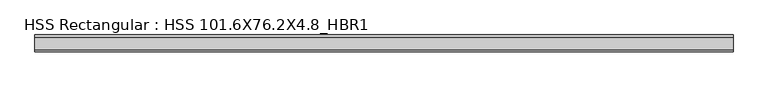
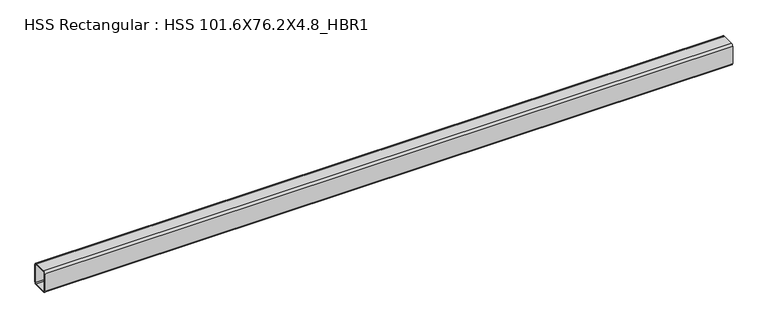
"""IFC4 building model written with IfcOpenShell, lengths in millimetres: beam geometry, HSS Rectangular : HSS 101.6X76.2X4.8_HBR1."""

import ifcopenshell
import ifcopenshell.guid

model = None  # the IFC model being written
_history = None  # IfcOwnerHistory: only IFC2X3 demands one
_inside = {}  # id of a spatial element -> (the spatial element, [elements in it])
_under = {}  # id of a project, library or spatial element -> (it, [spatial elements below it])
_declared = {}  # id of a project -> (the project, [libraries it declares])
_typed = {}  # id of a type object -> (the type object, [elements of that type])
_made_of = {}  # id of a material, layer set ... -> (it, [elements and type objects made of it])


def new_model(schema):
    """Start an empty IFC model of exactly this schema.

    Asked for "IFC4X3", IfcOpenShell would pick the latest addendum, in which some entities
    have other attributes; the version numbers below select the first issue.
    IFC2X3 requires an IfcOwnerHistory on every rooted entity: one is made here for all.
    """
    global model, _history
    if schema == "IFC4X3":
        model = ifcopenshell.file(schema_version=(4, 3, 0, 0))
    else:
        model = ifcopenshell.file(schema=schema)
    _inside.clear()
    _under.clear()
    _declared.clear()
    _typed.clear()
    _made_of.clear()
    _history = None
    if model.schema == "IFC2X3":
        org = make("IfcOrganization", Name="unknown")
        user = make(
            "IfcPersonAndOrganization",
            ThePerson=make("IfcPerson", FamilyName="unknown"),
            TheOrganization=org,
        )
        app = make(
            "IfcApplication",
            ApplicationDeveloper=org,
            Version="unknown",
            ApplicationFullName="unknown",
            ApplicationIdentifier="unknown",
        )
        _history = make(
            "IfcOwnerHistory",
            OwningUser=user,
            OwningApplication=app,
            ChangeAction="ADDED",
            CreationDate=0,
        )
    return model


def make(cls, **values):
    """One entity of the class cls with the attributes given. An attribute that is None is left unset."""
    return model.create_entity(
        cls, **{name: value for name, value in values.items() if value is not None}
    )


def rooted(cls, **values):
    """An entity with a GlobalId (a new one), such as an element, a storey or a relation."""
    return make(cls, GlobalId=ifcopenshell.guid.new(), OwnerHistory=_history, **values)


def si_unit(unit_type, name, prefix=None):
    """IfcSIUnit, for example si_unit("LENGTHUNIT", "METRE", prefix="MILLI")."""
    return make("IfcSIUnit", UnitType=unit_type, Prefix=prefix, Name=name)


def assignment(units):
    """IfcUnitAssignment: the units of a project."""
    return None if units is None else make("IfcUnitAssignment", Units=units)


def point(xyz):
    """IfcCartesianPoint."""
    return None if xyz is None else make("IfcCartesianPoint", Coordinates=xyz)


def direction(xyz):
    """IfcDirection."""
    return None if xyz is None else make("IfcDirection", DirectionRatios=xyz)


def frame(location, z_axis=None, x_axis=None):
    """IfcAxis2Placement3D, a coordinate frame: its origin and axes. An axis left out is left unset."""
    return make(
        "IfcAxis2Placement3D",
        Location=point(location),
        Axis=direction(z_axis),
        RefDirection=direction(x_axis),
    )


def frame_2d(location, x_axis=None):
    """IfcAxis2Placement2D, a coordinate frame in the plane: its origin and x axis."""
    return make(
        "IfcAxis2Placement2D", Location=point(location), RefDirection=direction(x_axis)
    )


def origin():
    """The frame at (0, 0, 0) with its axes left unset."""
    return frame((0.0, 0.0, 0.0))


def place(relative_to, where):
    """IfcLocalPlacement: puts the frame where relative to a parent placement (None: the world)."""
    return make(
        "IfcLocalPlacement", PlacementRelTo=relative_to, RelativePlacement=where
    )


def context(
    kind, dimensions, precision=None, world=None, true_north=None, identifier=None
):
    """IfcGeometricRepresentationContext, for example the 3D "Model" context."""
    return make(
        "IfcGeometricRepresentationContext",
        ContextIdentifier=identifier,
        ContextType=kind,
        CoordinateSpaceDimension=dimensions,
        Precision=precision,
        WorldCoordinateSystem=world,
        TrueNorth=true_north,
    )


def project(units=None, contexts=None):
    """IfcProject with its units and contexts."""
    return rooted(
        "IfcProject",
        Name="project",
        RepresentationContexts=contexts,
        UnitsInContext=assignment(units),
    )


def spatial(cls, under=None, at=None, **own):
    """A site, building, storey or space (cls), placed at a placement, below another one or the project."""
    s = rooted(cls, ObjectPlacement=at, **own)
    if under is not None:
        _under.setdefault(under.id(), (under, []))[1].append(s)
    return s


def polyline(points):
    """IfcPolyline through the points."""
    return make("IfcPolyline", Points=[point(p) for p in points])


def circle_curve(where, radius):
    """IfcCircle in the frame where."""
    return make("IfcCircle", Position=where, Radius=radius)


def trimmed(basis, trim1, trim2, sense, master):
    """IfcTrimmedCurve: the piece of a basis curve between two trims."""
    return make(
        "IfcTrimmedCurve",
        BasisCurve=basis,
        Trim1=trim1,
        Trim2=trim2,
        SenseAgreement=sense,
        MasterRepresentation=master,
    )


def segment(curve, same_sense, transition):
    """IfcCompositeCurveSegment."""
    return make(
        "IfcCompositeCurveSegment",
        Transition=transition,
        SameSense=same_sense,
        ParentCurve=curve,
    )


def composite_curve(segments, self_intersect=None):
    """IfcCompositeCurve: segments joined end to end."""
    return make("IfcCompositeCurve", Segments=segments, SelfIntersect=self_intersect)


def outline(outer, holes=None, kind="AREA"):
    """IfcArbitraryClosedProfileDef: a profile drawn as a closed curve; with holes, ...WithVoids."""
    if holes is None:
        return make("IfcArbitraryClosedProfileDef", ProfileType=kind, OuterCurve=outer)
    return make(
        "IfcArbitraryProfileDefWithVoids",
        ProfileType=kind,
        OuterCurve=outer,
        InnerCurves=holes,
    )


def extrude(swept, where, along, depth):
    """IfcExtrudedAreaSolid: the profile swept, set in the frame where, extruded along a direction by depth."""
    return make(
        "IfcExtrudedAreaSolid",
        SweptArea=swept,
        Position=where,
        ExtrudedDirection=direction(along),
        Depth=depth,
    )


def shape(context_of_items, identifier, shape_type, items):
    """IfcShapeRepresentation: the items that make up one representation, for example the "Body"."""
    return make(
        "IfcShapeRepresentation",
        ContextOfItems=context_of_items,
        RepresentationIdentifier=identifier,
        RepresentationType=shape_type,
        Items=items,
    )


def source(mapping_origin, context_of_items, identifier, shape_type, items):
    """IfcRepresentationMap: a shape defined once, which mapped items show again and again."""
    return make(
        "IfcRepresentationMap",
        MappingOrigin=mapping_origin,
        MappedRepresentation=shape(context_of_items, identifier, shape_type, items),
    )


def transform(
    local_origin,
    x_axis=None,
    y_axis=None,
    z_axis=None,
    scale=None,
    scale2=None,
    scale3=None,
    uniform=True,
):
    """IfcCartesianTransformationOperator3D, or its non-uniform kind. x_axis, y_axis, z_axis: its Axis1, 2, 3."""
    if uniform:
        return make(
            "IfcCartesianTransformationOperator3D",
            Axis1=direction(x_axis),
            Axis2=direction(y_axis),
            LocalOrigin=point(local_origin),
            Scale=scale,
            Axis3=direction(z_axis),
        )
    return make(
        "IfcCartesianTransformationOperator3DnonUniform",
        Axis1=direction(x_axis),
        Axis2=direction(y_axis),
        LocalOrigin=point(local_origin),
        Scale=scale,
        Axis3=direction(z_axis),
        Scale2=scale2,
        Scale3=scale3,
    )


def mapped(mapping_source, mapping_target):
    """IfcMappedItem: shows the shape of a source again, moved by a transform."""
    return make(
        "IfcMappedItem", MappingSource=mapping_source, MappingTarget=mapping_target
    )


def made_of(thing, what):
    """Note that an element or type object is made of a material, layer set ...; save() writes the relation."""
    if what is not None:
        _made_of.setdefault(what.id(), (what, []))[1].append(thing)
    return thing


def element(
    cls,
    number,
    at=None,
    inside=None,
    cuts=None,
    type_object=None,
    material=None,
    context=None,
    identifier="Body",
    shape_type=None,
    held_by="IfcProductDefinitionShape",
    body=None,
    shapes=None,
    **own,
):
    """One element of the class cls, such as IfcWall. Its Tag is "e" and its number.

    at: its placement. inside: the storey or other place that contains it. cuts: it is an
    opening in that element (IfcRelVoidsElement). A single representation is given by context,
    identifier, shape_type and body (its items); several are given by shapes. held_by: the class
    of the entity that holds the representations. save() writes the other relations.
    """
    e = rooted(cls, Tag="e%d" % number, ObjectPlacement=at, **own)
    if body is not None:
        shapes = [shape(context, identifier, shape_type, body)]
    if shapes is not None:
        e.Representation = make(held_by, Representations=shapes)
    if inside is not None:
        _inside.setdefault(inside.id(), (inside, []))[1].append(e)
    if cuts is not None:
        rooted(
            "IfcRelVoidsElement", RelatingBuildingElement=cuts, RelatedOpeningElement=e
        )
    if type_object is not None:
        _typed.setdefault(type_object.id(), (type_object, []))[1].append(e)
    return made_of(e, material)


def aggregate(whole, parts):
    """IfcRelAggregates: a whole, such as a stair, and the parts it consists of."""
    return rooted("IfcRelAggregates", RelatingObject=whole, RelatedObjects=parts)


def save(model, path):
    """Write the relations noted so far, then the file.

    IfcRelAggregates (storeys below a building ...), IfcRelContainedInSpatialStructure (elements
    in a storey), IfcRelDefinesByType, IfcRelAssociatesMaterial and IfcRelDeclares: one each for
    every whole, place, type object, material and project.
    """
    for whole, parts in _under.values():
        aggregate(whole, parts)
    for where, things in _inside.values():
        rooted(
            "IfcRelContainedInSpatialStructure",
            RelatedElements=things,
            RelatingStructure=where,
        )
    for kind, things in _typed.values():
        rooted("IfcRelDefinesByType", RelatedObjects=things, RelatingType=kind)
    for what, things in _made_of.values():
        rooted("IfcRelAssociatesMaterial", RelatedObjects=things, RelatingMaterial=what)
    for by, libraries in _declared.values():
        rooted("IfcRelDeclares", RelatingContext=by, RelatedDefinitions=libraries)
    model.write(path)


def hss_rectangular_hss_101_6x76_2x4_8_hbr1_9f14be74(model_context):
    return source(origin(), model_context, "Body", "SweptSolid", [
        extrude(outline(composite_curve([segment(polyline([(38.1, 41.275), (38.1, -41.275)]), True, "CONTINUOUS"), segment(trimmed(circle_curve(frame_2d((28.575, -41.275)), 9.525), [point((38.1, -41.275))], [point((28.575, -50.8))], False, "CARTESIAN"), True, "CONTINUOUS"), segment(polyline([(28.575, -50.8), (-28.575, -50.8)]), True, "CONTINUOUS"), segment(trimmed(circle_curve(frame_2d((-28.575, -41.275)), 9.525), [point((-28.575, -50.8))], [point((-38.1, -41.275))], False, "CARTESIAN"), True, "CONTINUOUS"), segment(polyline([(-38.1, -41.275), (-38.1, 41.275)]), True, "CONTINUOUS"), segment(trimmed(circle_curve(frame_2d((-28.575, 41.275)), 9.525), [point((-38.1, 41.275))], [point((-28.575, 50.8))], False, "CARTESIAN"), True, "CONTINUOUS"), segment(polyline([(-28.575, 50.8), (28.575, 50.8)]), True, "CONTINUOUS"), segment(trimmed(circle_curve(frame_2d((28.575, 41.275)), 9.525), [point((28.575, 50.8))], [point((38.1, 41.275))], False, "CARTESIAN"), True, "CONTINUOUS")], self_intersect=False), holes=[composite_curve([segment(trimmed(circle_curve(frame_2d((-28.575, 41.275)), 4.7625), [point((-28.575, 46.0375))], [point((-33.3375, 41.275))], True, "CARTESIAN"), True, "CONTINUOUS"), segment(polyline([(-33.3375, 41.275), (-33.3375, -41.275)]), True, "CONTINUOUS"), segment(trimmed(circle_curve(frame_2d((-28.575, -41.275)), 4.7625), [point((-33.3375, -41.275))], [point((-28.575, -46.0375))], True, "CARTESIAN"), True, "CONTINUOUS"), segment(polyline([(-28.575, -46.0375), (28.575, -46.0375)]), True, "CONTINUOUS"), segment(trimmed(circle_curve(frame_2d((28.575, -41.275)), 4.7625), [point((28.575, -46.0375))], [point((33.3375, -41.275))], True, "CARTESIAN"), True, "CONTINUOUS"), segment(polyline([(33.3375, -41.275), (33.3375, 41.275)]), True, "CONTINUOUS"), segment(trimmed(circle_curve(frame_2d((28.575, 41.275)), 4.7625), [point((33.3375, 41.275))], [point((28.575, 46.0375))], True, "CARTESIAN"), True, "CONTINUOUS"), segment(polyline([(28.575, 46.0375), (-28.575, 46.0375)]), True, "CONTINUOUS")], self_intersect=False)]), frame((-1531.628843, 0.0, 0.0), z_axis=(1.0, 0.0, 0.0), x_axis=(0.0, 1.0, 0.0)), (0.0, 0.0, 1.0), 3138.6008181),
    ])


if __name__ == "__main__":
    model = new_model("IFC4")
    model_context = context("Model", 3, world=origin())
    ifc_project = project(units=[si_unit("LENGTHUNIT", "METRE", prefix="MILLI")], contexts=[model_context])
    site = spatial("IfcSite", under=ifc_project)
    building = spatial("IfcBuilding", under=site)
    placement = place(None, origin())
    hss_rectangular_hss_101_6x76_2x4_8_hbr1_shape = hss_rectangular_hss_101_6x76_2x4_8_hbr1_9f14be74(model_context)
    element("IfcBeam", 1, ObjectType="HSS Rectangular : HSS 101.6X76.2X4.8_HBR1", at=placement, inside=building, context=model_context, shape_type="MappedRepresentation", body=[
        mapped(hss_rectangular_hss_101_6x76_2x4_8_hbr1_shape, transform((0.0, 0.0, 0.0), x_axis=(1.0, 0.0, 0.0), y_axis=(0.0, 1.0, 0.0), z_axis=(0.0, 0.0, 1.0))),
    ])
    save(model, "model.ifc")

# Revit data of these elements
# Type "HSS Rectangular : HSS 101.6X76.2X4.8_HBR1"
#   Section Name Key = "HSS 4X3X3/16"
#   Assembly Code = "B10"
#   Width = 7.62 cm
#   Wall Nominal Thickness = 0.4763 cm
#   Wall Design Thickness = 0.442 cm
#   Torsional Moment of Inertia = 260.561 cm⁴
#   Torsional Modulus = 61.2876 cm³
#   Section Area = 14.4516 cm²
#   Plastic Modulus weak axis = 40.3122 cm³
#   Plastic Modulus strong axis = 49.1612 cm³
#   Perimeter = 0.881482 m²/m
#   Outer Fillet = 0.9525 cm
#   Nominal Weight = 12.1285 kgf/m
#   Moment of Inertia weak axis = 131.529 cm⁴
#   Moment of Inertia strong axis = 205.202 cm⁴
#   Inner Fillet = 0.4763 cm
#   Height = 10.16 cm
#   Elastic Modulus weak axis = 34.4128 cm³
#   Elastic Modulus strong axis = 40.476 cm³
#   Centroid Vertical = 5.08 cm
#   Centroid Horizontal = 3.81 cm
#   Length [instance default] = 1524 mm
#   Structural Material [instance default] = Steel ASTM A500, Grade B, Rectangular and Square
#   Principal Axes Angle = 0
# Element 1 (IfcBeam, "HSS Rectangular : HSS 101.6X76.2X4.8_HBR1")
#   Structural Material = Steel ASTM A992
#   Materials on its faces: "Steel ASTM A992"
# Materials
#   "Steel ASTM A500, Grade B, Rectangular and Square": class "Metal", colour RGB 199 199 199, transparency 0, Description = "Carbon steel", Cost = 0
#   "Steel ASTM A992": class "Metal", colour RGB 199 199 199, transparency 0, Description = "Structural steel 50ksi", Cost = 0
